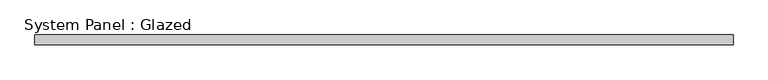
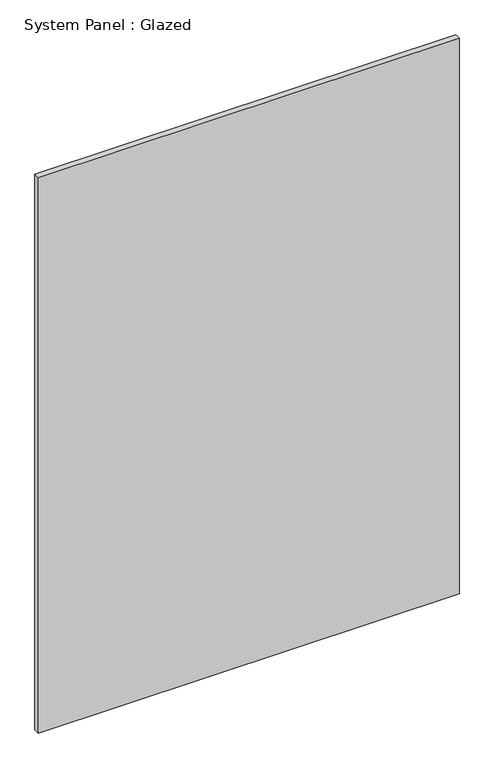
"""IFC4 building model written with IfcOpenShell, lengths in millimetres: plate geometry, System Panel : Glazed."""

from ifc_helpers import new_model, si_unit, origin, origin_with_axes, place, context, project, spatial, polyline, outline, extrude, source, transform, mapped, element, save


def system_panel_glazed_ccadeef2(model_context):
    return source(origin(), model_context, "Body", "SweptSolid", [
        extrude(outline(polyline([(877.5, -49.5), (-877.5, -49.5), (-877.5, -24.5), (877.5, -24.5), (877.5, -49.5)])), origin_with_axes(), (0.0, 0.0, 1.0), 2450.0),
    ])


if __name__ == "__main__":
    model = new_model("IFC4")
    model_context = context("Model", 3, world=origin())
    ifc_project = project(units=[si_unit("LENGTHUNIT", "METRE", prefix="MILLI")], contexts=[model_context])
    site = spatial("IfcSite", under=ifc_project)
    building = spatial("IfcBuilding", under=site)
    placement = place(None, origin())
    system_panel_glazed_shape = system_panel_glazed_ccadeef2(model_context)
    element("IfcPlate", 1, ObjectType="System Panel : Glazed", at=placement, inside=building, context=model_context, shape_type="MappedRepresentation", body=[
        mapped(system_panel_glazed_shape, transform((0.0, 0.0, 0.0), x_axis=(1.0, 0.0, 0.0), y_axis=(0.0, 1.0, 0.0), z_axis=(0.0, 0.0, 1.0))),
    ])
    save(model, "model.ifc")

# Revit data of these elements
# Type "System Panel : Glazed"
#   Keynote = "H11"
#   Construction Type Id = "GSP4R"
#   Analytic Construction = "1/8 in Pilkington single glazing"
#   Visual Light Transmittance = 0.9
#   Solar Heat Gain Coefficient = 0.86
#   Heat Transfer Coefficient (U) = 6.7069 W/(m²·K)
# Element 1 (IfcPlate, "System Panel : Glazed")
#   Materials on its faces: "Glass"
# Materials
#   "Glass": class "Glass", colour RGB 0 128 192, transparency 0.9, Description = "Soda Lime Glass", Cost = 0
